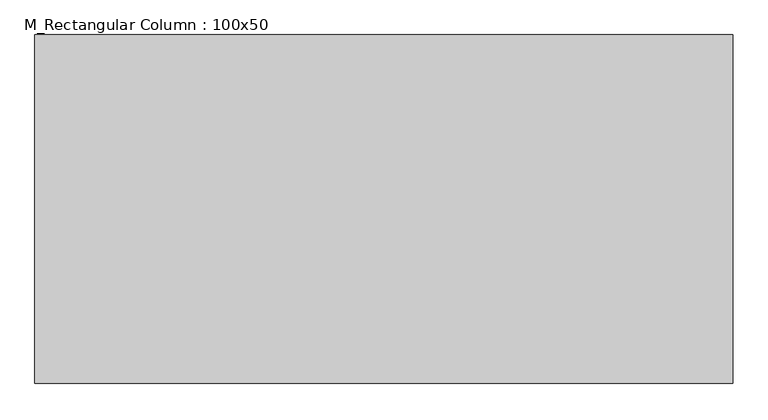
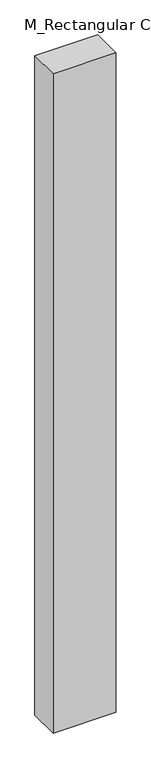
"""IFC4 building model written with IfcOpenShell, lengths in millimetres: column geometry, M_Rectangular Column : 100x50."""

from ifc_helpers import new_model, si_unit, frame, origin, place, context, project, spatial, polyline, outline, extrude, source, transform, mapped, element, save


def m_rectangular_column_100x50_89a3459c(model_context):
    return source(origin(), model_context, "Body", "SweptSolid", [
        extrude(outline(polyline([(500.0, 250.0), (500.0, -250.0), (-500.0, -250.0), (-500.0, 250.0), (500.0, 250.0)])), frame((0.0, 0.0, -3200.0), z_axis=(0.0, 0.0, 1.0), x_axis=(1.0, 0.0, 0.0)), (0.0, 0.0, 1.0), 11100.0),
    ])


if __name__ == "__main__":
    model = new_model("IFC4")
    model_context = context("Model", 3, world=origin())
    ifc_project = project(units=[si_unit("LENGTHUNIT", "METRE", prefix="MILLI")], contexts=[model_context])
    site = spatial("IfcSite", under=ifc_project)
    building = spatial("IfcBuilding", under=site)
    placement = place(None, origin())
    m_rectangular_column_100x50_shape = m_rectangular_column_100x50_89a3459c(model_context)
    element("IfcColumn", 1, ObjectType="M_Rectangular Column : 100x50", at=placement, inside=building, context=model_context, shape_type="MappedRepresentation", body=[
        mapped(m_rectangular_column_100x50_shape, transform((0.0, 0.0, 0.0), x_axis=(1.0, 0.0, 0.0), y_axis=(0.0, 1.0, 0.0), z_axis=(0.0, 0.0, 1.0))),
    ])
    save(model, "model.ifc")

# Revit data of these elements
# Type "M_Rectangular Column : 100x50"
#   Depth = 50 cm
#   Offset Base = 0 cm
#   Offset Top = 0 cm
#   Width = 100 cm
#   Material = none
